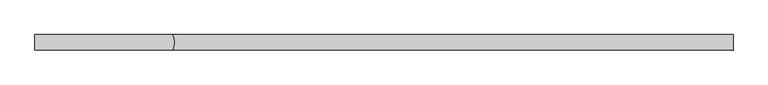
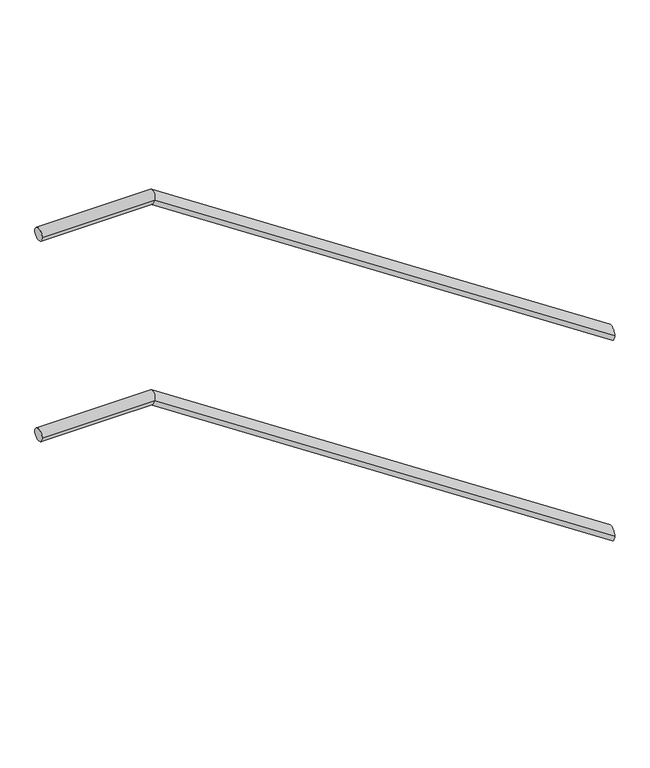
"""IFC4 building model written with IfcOpenShell, lengths in millimetres: railing geometry."""

import ifcopenshell
import ifcopenshell.guid

model = None  # the IFC model being written
_history = None  # IfcOwnerHistory: only IFC2X3 demands one
_inside = {}  # id of a spatial element -> (the spatial element, [elements in it])
_under = {}  # id of a project, library or spatial element -> (it, [spatial elements below it])
_declared = {}  # id of a project -> (the project, [libraries it declares])
_typed = {}  # id of a type object -> (the type object, [elements of that type])
_made_of = {}  # id of a material, layer set ... -> (it, [elements and type objects made of it])


def new_model(schema):
    """Start an empty IFC model of exactly this schema.

    Asked for "IFC4X3", IfcOpenShell would pick the latest addendum, in which some entities
    have other attributes; the version numbers below select the first issue.
    IFC2X3 requires an IfcOwnerHistory on every rooted entity: one is made here for all.
    """
    global model, _history
    if schema == "IFC4X3":
        model = ifcopenshell.file(schema_version=(4, 3, 0, 0))
    else:
        model = ifcopenshell.file(schema=schema)
    _inside.clear()
    _under.clear()
    _declared.clear()
    _typed.clear()
    _made_of.clear()
    _history = None
    if model.schema == "IFC2X3":
        org = make("IfcOrganization", Name="unknown")
        user = make(
            "IfcPersonAndOrganization",
            ThePerson=make("IfcPerson", FamilyName="unknown"),
            TheOrganization=org,
        )
        app = make(
            "IfcApplication",
            ApplicationDeveloper=org,
            Version="unknown",
            ApplicationFullName="unknown",
            ApplicationIdentifier="unknown",
        )
        _history = make(
            "IfcOwnerHistory",
            OwningUser=user,
            OwningApplication=app,
            ChangeAction="ADDED",
            CreationDate=0,
        )
    return model


def make(cls, **values):
    """One entity of the class cls with the attributes given. An attribute that is None is left unset."""
    return model.create_entity(
        cls, **{name: value for name, value in values.items() if value is not None}
    )


def rooted(cls, **values):
    """An entity with a GlobalId (a new one), such as an element, a storey or a relation."""
    return make(cls, GlobalId=ifcopenshell.guid.new(), OwnerHistory=_history, **values)


def si_unit(unit_type, name, prefix=None):
    """IfcSIUnit, for example si_unit("LENGTHUNIT", "METRE", prefix="MILLI")."""
    return make("IfcSIUnit", UnitType=unit_type, Prefix=prefix, Name=name)


def assignment(units):
    """IfcUnitAssignment: the units of a project."""
    return None if units is None else make("IfcUnitAssignment", Units=units)


def point(xyz):
    """IfcCartesianPoint."""
    return None if xyz is None else make("IfcCartesianPoint", Coordinates=xyz)


def direction(xyz):
    """IfcDirection."""
    return None if xyz is None else make("IfcDirection", DirectionRatios=xyz)


def frame(location, z_axis=None, x_axis=None):
    """IfcAxis2Placement3D, a coordinate frame: its origin and axes. An axis left out is left unset."""
    return make(
        "IfcAxis2Placement3D",
        Location=point(location),
        Axis=direction(z_axis),
        RefDirection=direction(x_axis),
    )


def origin():
    """The frame at (0, 0, 0) with its axes left unset."""
    return frame((0.0, 0.0, 0.0))


def place(relative_to, where):
    """IfcLocalPlacement: puts the frame where relative to a parent placement (None: the world)."""
    return make(
        "IfcLocalPlacement", PlacementRelTo=relative_to, RelativePlacement=where
    )


def context(
    kind, dimensions, precision=None, world=None, true_north=None, identifier=None
):
    """IfcGeometricRepresentationContext, for example the 3D "Model" context."""
    return make(
        "IfcGeometricRepresentationContext",
        ContextIdentifier=identifier,
        ContextType=kind,
        CoordinateSpaceDimension=dimensions,
        Precision=precision,
        WorldCoordinateSystem=world,
        TrueNorth=true_north,
    )


def project(units=None, contexts=None):
    """IfcProject with its units and contexts."""
    return rooted(
        "IfcProject",
        Name="project",
        RepresentationContexts=contexts,
        UnitsInContext=assignment(units),
    )


def spatial(cls, under=None, at=None, **own):
    """A site, building, storey or space (cls), placed at a placement, below another one or the project."""
    s = rooted(cls, ObjectPlacement=at, **own)
    if under is not None:
        _under.setdefault(under.id(), (under, []))[1].append(s)
    return s


def circle_curve(where, radius):
    """IfcCircle in the frame where."""
    return make("IfcCircle", Position=where, Radius=radius)


def ellipse_curve(where, semi_axis1, semi_axis2):
    """IfcEllipse in the frame where."""
    return make(
        "IfcEllipse", Position=where, SemiAxis1=semi_axis1, SemiAxis2=semi_axis2
    )


def shape(context_of_items, identifier, shape_type, items):
    """IfcShapeRepresentation: the items that make up one representation, for example the "Body"."""
    return make(
        "IfcShapeRepresentation",
        ContextOfItems=context_of_items,
        RepresentationIdentifier=identifier,
        RepresentationType=shape_type,
        Items=items,
    )


def source(mapping_origin, context_of_items, identifier, shape_type, items):
    """IfcRepresentationMap: a shape defined once, which mapped items show again and again."""
    return make(
        "IfcRepresentationMap",
        MappingOrigin=mapping_origin,
        MappedRepresentation=shape(context_of_items, identifier, shape_type, items),
    )


def transform(
    local_origin,
    x_axis=None,
    y_axis=None,
    z_axis=None,
    scale=None,
    scale2=None,
    scale3=None,
    uniform=True,
):
    """IfcCartesianTransformationOperator3D, or its non-uniform kind. x_axis, y_axis, z_axis: its Axis1, 2, 3."""
    if uniform:
        return make(
            "IfcCartesianTransformationOperator3D",
            Axis1=direction(x_axis),
            Axis2=direction(y_axis),
            LocalOrigin=point(local_origin),
            Scale=scale,
            Axis3=direction(z_axis),
        )
    return make(
        "IfcCartesianTransformationOperator3DnonUniform",
        Axis1=direction(x_axis),
        Axis2=direction(y_axis),
        LocalOrigin=point(local_origin),
        Scale=scale,
        Axis3=direction(z_axis),
        Scale2=scale2,
        Scale3=scale3,
    )


def mapped(mapping_source, mapping_target):
    """IfcMappedItem: shows the shape of a source again, moved by a transform."""
    return make(
        "IfcMappedItem", MappingSource=mapping_source, MappingTarget=mapping_target
    )


def made_of(thing, what):
    """Note that an element or type object is made of a material, layer set ...; save() writes the relation."""
    if what is not None:
        _made_of.setdefault(what.id(), (what, []))[1].append(thing)
    return thing


def element(
    cls,
    number,
    at=None,
    inside=None,
    cuts=None,
    type_object=None,
    material=None,
    context=None,
    identifier="Body",
    shape_type=None,
    held_by="IfcProductDefinitionShape",
    body=None,
    shapes=None,
    **own,
):
    """One element of the class cls, such as IfcWall. Its Tag is "e" and its number.

    at: its placement. inside: the storey or other place that contains it. cuts: it is an
    opening in that element (IfcRelVoidsElement). A single representation is given by context,
    identifier, shape_type and body (its items); several are given by shapes. held_by: the class
    of the entity that holds the representations. save() writes the other relations.
    """
    e = rooted(cls, Tag="e%d" % number, ObjectPlacement=at, **own)
    if body is not None:
        shapes = [shape(context, identifier, shape_type, body)]
    if shapes is not None:
        e.Representation = make(held_by, Representations=shapes)
    if inside is not None:
        _inside.setdefault(inside.id(), (inside, []))[1].append(e)
    if cuts is not None:
        rooted(
            "IfcRelVoidsElement", RelatingBuildingElement=cuts, RelatedOpeningElement=e
        )
    if type_object is not None:
        _typed.setdefault(type_object.id(), (type_object, []))[1].append(e)
    return made_of(e, material)


def aggregate(whole, parts):
    """IfcRelAggregates: a whole, such as a stair, and the parts it consists of."""
    return rooted("IfcRelAggregates", RelatingObject=whole, RelatedObjects=parts)


def save(model, path):
    """Write the relations noted so far, then the file.

    IfcRelAggregates (storeys below a building ...), IfcRelContainedInSpatialStructure (elements
    in a storey), IfcRelDefinesByType, IfcRelAssociatesMaterial and IfcRelDeclares: one each for
    every whole, place, type object, material and project.
    """
    for whole, parts in _under.values():
        aggregate(whole, parts)
    for where, things in _inside.values():
        rooted(
            "IfcRelContainedInSpatialStructure",
            RelatedElements=things,
            RelatingStructure=where,
        )
    for kind, things in _typed.values():
        rooted("IfcRelDefinesByType", RelatedObjects=things, RelatingType=kind)
    for what, things in _made_of.values():
        rooted("IfcRelAssociatesMaterial", RelatedObjects=things, RelatingMaterial=what)
    for by, libraries in _declared.values():
        rooted("IfcRelDeclares", RelatingContext=by, RelatedDefinitions=libraries)
    model.write(path)


def plane_surface(at):
    """IfcPlane: the flat surface through the origin of the frame at, square to its z axis."""
    return make("IfcPlane", Position=at)


def cylinder_surface(at, radius):
    """IfcCylindricalSurface: all points at the distance radius from the z axis of the frame at."""
    return make("IfcCylindricalSurface", Position=at, Radius=radius)


def advanced_brep(points, edges, surfaces, faces):
    """IfcAdvancedBrep: a solid bounded by faces that lie on surfaces and meet in shared edges.

    An edge is (start, end): straight between two places in points (the first is 0);
    or (start, end, curve); or (start, end, curve, False) where it runs against its curve.
    A face is (place in surfaces, loops), or (place, loops, False) where it looks against
    its surface's normal. A loop lists edges by number (the first is 1), with a minus sign
    where the edge is run from its end to its start. The first loop is the outer one.
    """
    corners = [point(p) for p in points]
    vertices = [make("IfcVertexPoint", VertexGeometry=c) for c in corners]
    made = []
    for start, end, *more in edges:
        made.append(
            make(
                "IfcEdgeCurve",
                EdgeStart=vertices[start],
                EdgeEnd=vertices[end],
                EdgeGeometry=more[0] if more else make("IfcPolyline", Points=[corners[start], corners[end]]),
                SameSense=more[1] if len(more) > 1 else True,
            )
        )
    hull = []
    for where, loops, *sense in faces:
        bounds = []
        for j, loop in enumerate(loops):
            ring = [make("IfcOrientedEdge", EdgeElement=made[abs(k) - 1], Orientation=k > 0) for k in loop]
            bounds.append(
                make(
                    "IfcFaceOuterBound" if j == 0 else "IfcFaceBound",
                    Bound=make("IfcEdgeLoop", EdgeList=ring),
                    Orientation=True,
                )
            )
        hull.append(make("IfcAdvancedFace", Bounds=bounds, FaceSurface=surfaces[where], SameSense=sense[0] if sense else True))
    return make("IfcAdvancedBrep", Outer=make("IfcClosedShell", CfsFaces=hull))


def railing_36ed9c91(model_context):
    return source(origin(), model_context, "Body", "AdvancedBrep", [
        advanced_brep(
        [(48078.2332408, 8219.6306666, 910.5875748), (48078.2332408, 8249.6306666, 910.5875748), (46993.7216539, 8219.6306666, 1627.8571429), (46993.7216539, 8249.6306666, 1627.8571429), (46728.2332408, 8219.6306666, 1627.8571429), (46728.2332408, 8249.6306666, 1627.8571429)],
        [
            (0, 1, ellipse_curve(frame((48078.2332408, 8234.6306666, 910.5875748), z_axis=(1.0, 0.0, 0.0), x_axis=(0.0, 0.0, -1.0)), 17.9838538, 15.0)),
            (1, 0, ellipse_curve(frame((48078.2332408, 8234.6306666, 910.5875748), z_axis=(1.0, 0.0, 0.0), x_axis=(0.0, 0.0, -1.0)), 17.9838538, 15.0)),
            (0, 2),
            (2, 3, ellipse_curve(frame((46993.7216539, 8234.6306666, 1627.8571429), z_axis=(0.9576224501515418, 0.0, -0.28802646226650325), x_axis=(-0.288026462266502, 0.0, -0.9576224501515423)), 15.6637932, 15.0)),
            (3, 1),
            (3, 2, ellipse_curve(frame((46993.7216539, 8234.6306666, 1627.8571429), z_axis=(0.9576224501515418, 0.0, -0.28802646226650325), x_axis=(-0.288026462266502, 0.0, -0.9576224501515423)), 15.6637932, 15.0)),
            (4, 5, circle_curve(frame((46728.2332408, 8234.6306666, 1627.8571429), z_axis=(-1.0, 0.0, 0.0), x_axis=(0.0, 1.0, 0.0)), 15.0)),
            (5, 4, circle_curve(frame((46728.2332408, 8234.6306666, 1627.8571429), z_axis=(-1.0, 0.0, 0.0), x_axis=(0.0, 1.0, 0.0)), 15.0)),
            (2, 4),
            (5, 3),
        ],
        [
            plane_surface(frame((48078.2332408, 8234.6306666, 928.5714286), z_axis=(1.0, 0.0, 0.0), x_axis=(0.0, -1.0, 0.0))),
            cylinder_surface(frame((48069.9586226, 8234.6306666, 916.0602059), z_axis=(0.8340815140684851, 0.0, -0.5516412130082591), x_axis=(0.0, 1.0, 0.0)), 15.0),
            plane_surface(frame((46728.2332408, 8234.6306666, 1642.8571429), z_axis=(-1.0, 0.0, 0.0), x_axis=(0.0, -1.0, 0.0))),
            cylinder_surface(frame((46998.2332408, 8234.6306666, 1627.8571429), z_axis=(1.0, 0.0, 0.0), x_axis=(0.0, 1.0, 0.0)), 15.0),
        ],
        [
            (0, [[1, 2]]),
            (1, [[-1, 3, 4, 5]]),
            (1, [[-2, -5, 6, -3]]),
            (2, [[7, 8]]),
            (3, [[-4, 9, -8, 10]]),
            (3, [[-6, -10, -7, -9]]),
        ],
    ),
        advanced_brep(
        [(48078.2332408, 8219.6306666, 1410.5875748), (48078.2332408, 8249.6306666, 1410.5875748), (46993.7216539, 8219.6306666, 2127.8571429), (46993.7216539, 8249.6306666, 2127.8571429), (46728.2332408, 8219.6306666, 2127.8571429), (46728.2332408, 8249.6306666, 2127.8571429)],
        [
            (0, 1, ellipse_curve(frame((48078.2332408, 8234.6306666, 1410.5875748), z_axis=(1.0, 0.0, 0.0), x_axis=(0.0, 0.0, -1.0)), 17.9838538, 15.0)),
            (1, 0, ellipse_curve(frame((48078.2332408, 8234.6306666, 1410.5875748), z_axis=(1.0, 0.0, 0.0), x_axis=(0.0, 0.0, -1.0)), 17.9838538, 15.0)),
            (0, 2),
            (2, 3, ellipse_curve(frame((46993.7216539, 8234.6306666, 2127.8571429), z_axis=(0.9576224501515418, 0.0, -0.28802646226650325), x_axis=(-0.288026462266502, 0.0, -0.9576224501515423)), 15.6637932, 15.0)),
            (3, 1),
            (3, 2, ellipse_curve(frame((46993.7216539, 8234.6306666, 2127.8571429), z_axis=(0.9576224501515418, 0.0, -0.28802646226650325), x_axis=(-0.288026462266502, 0.0, -0.9576224501515423)), 15.6637932, 15.0)),
            (4, 5, circle_curve(frame((46728.2332408, 8234.6306666, 2127.8571429), z_axis=(-1.0, 0.0, 0.0), x_axis=(0.0, 1.0, 0.0)), 15.0)),
            (5, 4, circle_curve(frame((46728.2332408, 8234.6306666, 2127.8571429), z_axis=(-1.0, 0.0, 0.0), x_axis=(0.0, 1.0, 0.0)), 15.0)),
            (2, 4),
            (5, 3),
        ],
        [
            plane_surface(frame((48078.2332408, 8234.6306666, 1428.5714286), z_axis=(1.0, 0.0, 0.0), x_axis=(0.0, -1.0, 0.0))),
            cylinder_surface(frame((48069.9586226, 8234.6306666, 1416.0602059), z_axis=(0.8340815140684851, 0.0, -0.5516412130082591), x_axis=(0.0, 1.0, 0.0)), 15.0),
            plane_surface(frame((46728.2332408, 8234.6306666, 2142.8571429), z_axis=(-1.0, 0.0, 0.0), x_axis=(0.0, -1.0, 0.0))),
            cylinder_surface(frame((46998.2332408, 8234.6306666, 2127.8571429), z_axis=(1.0, 0.0, 0.0), x_axis=(0.0, 1.0, 0.0)), 15.0),
        ],
        [
            (0, [[1, 2]]),
            (1, [[-1, 3, 4, 5]]),
            (1, [[-2, -5, 6, -3]]),
            (2, [[7, 8]]),
            (3, [[-4, 9, -8, 10]]),
            (3, [[-6, -10, -7, -9]]),
        ],
    ),
    ])


if __name__ == "__main__":
    model = new_model("IFC4")
    model_context = context("Model", 3, world=origin())
    ifc_project = project(units=[si_unit("LENGTHUNIT", "METRE", prefix="MILLI")], contexts=[model_context])
    site = spatial("IfcSite", under=ifc_project)
    building = spatial("IfcBuilding", under=site)
    placement = place(None, origin())
    railing_shape = railing_36ed9c91(model_context)
    element("IfcRailing", 1, at=placement, inside=building, context=model_context, shape_type="MappedRepresentation", body=[
        mapped(railing_shape, transform((0.0, 0.0, 0.0), x_axis=(1.0, 0.0, 0.0), y_axis=(0.0, 1.0, 0.0), z_axis=(0.0, 0.0, 1.0))),
    ])
    save(model, "model.ifc")
